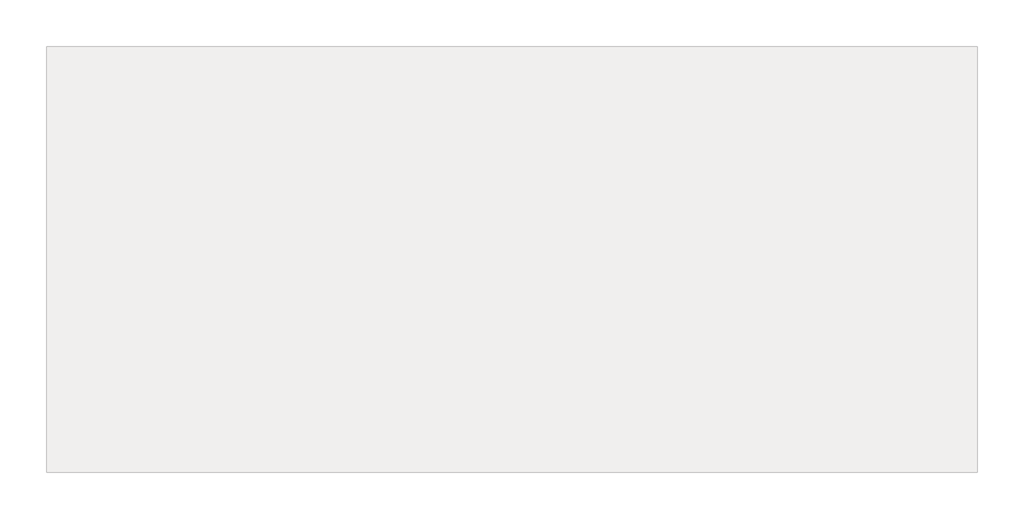
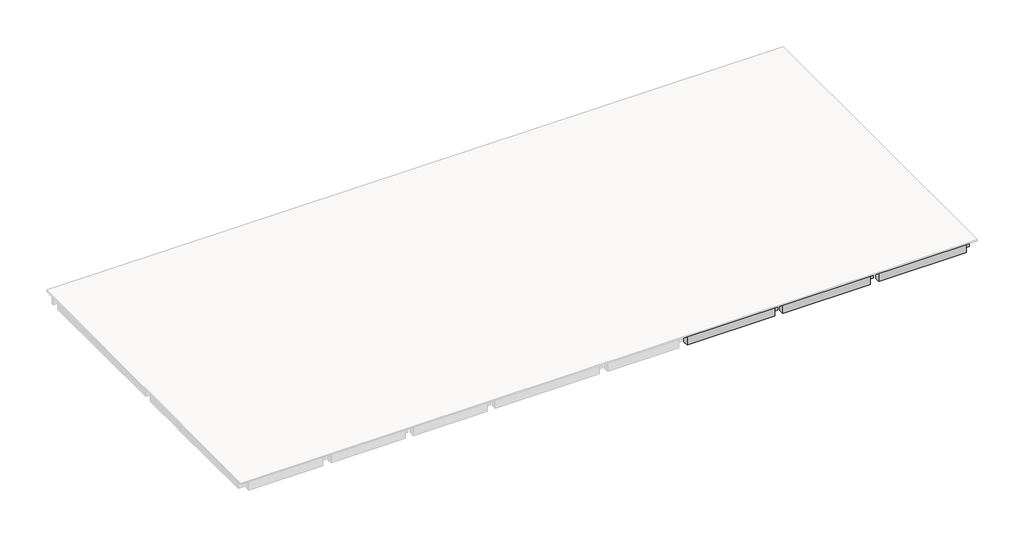
# One storey, part 2 of 2: 30 beams.
"""IFC4 building model written with IfcOpenShell, lengths in millimetres."""

from ifc_helpers import new_model, si_unit, frame, origin, place, context, project, spatial, polyline, outline, extrude, faceted_brep, element, save

model = new_model("IFC4")

# Units and contexts
model_context = context("Model", 3, world=origin())
ifc_project = project(units=[si_unit("LENGTHUNIT", "METRE", prefix="MILLI")], contexts=[model_context])

# Site, building, storey
site = spatial("IfcSite", under=ifc_project)
building = spatial("IfcBuilding", under=site)
storey = spatial("IfcBuildingStorey", under=building, Name="TOC", Elevation=7650.0)

# Beams
placement = place(None, origin())
element("IfcBeam", 1, ObjectType="RC Beam_Rectangular : H_SB_ACB_B400xH900", at=placement, inside=storey, context=model_context, shape_type="Brep", body=[
    faceted_brep([(39124.7, 12116.5208589, 6750.0), (39124.7, 12116.5208589, 7549.0), (38724.7, 12116.5208589, 7549.0), (32124.7, 12116.5208589, 7549.0), (32124.7, 12116.5208589, 6750.0), (38724.7, 12116.5208589, 6750.0), (39124.7, 12516.5208589, 6750.0), (32124.7, 12516.5208589, 6750.0), (38724.7, 12516.5208589, 6750.0), (39124.7, 12516.5208589, 7549.0), (32124.7, 12516.5208589, 7549.0), (38724.7, 12516.5208589, 7549.0)], [[[0, 1, 2, 3, 4, 5]], [[6, 0, 5, 4, 7, 8]], [[9, 6, 8, 7, 10, 11]], [[1, 9, 11, 10, 3, 2]], [[0, 6, 9, 1]], [[4, 3, 10, 7]]]),
])
element("IfcBeam", 2, ObjectType="RC Beam_Rectangular : H_SB_ACB_B400xH900", at=placement, inside=storey, context=model_context, shape_type="Brep", body=[
    faceted_brep([(46124.7, 12116.5208589, 6750.0), (46124.7, 12116.5208589, 7549.0), (45724.7, 12116.5208589, 7549.0), (39124.7, 12116.5208589, 7549.0), (39124.7, 12116.5208589, 6750.0), (45724.7, 12116.5208589, 6750.0), (46124.7, 12516.5208589, 6750.0), (39124.7, 12516.5208589, 6750.0), (45724.7, 12516.5208589, 6750.0), (46124.7, 12516.5208589, 7549.0), (39124.7, 12516.5208589, 7549.0), (45724.7, 12516.5208589, 7549.0)], [[[0, 1, 2, 3, 4, 5]], [[6, 0, 5, 4, 7, 8]], [[9, 6, 8, 7, 10, 11]], [[1, 9, 11, 10, 3, 2]], [[0, 6, 9, 1]], [[4, 3, 10, 7]]]),
])
element("IfcBeam", 3, ObjectType="RC Beam_Rectangular : H_SB_ACB_B400xH900", at=placement, inside=storey, context=model_context, shape_type="Brep", body=[
    faceted_brep([(53124.7, 12116.5208589, 6750.0), (53124.7, 12116.5208589, 7549.0), (52724.7, 12116.5208589, 7549.0), (46124.7, 12116.5208589, 7549.0), (46124.7, 12116.5208589, 6750.0), (52724.7, 12116.5208589, 6750.0), (53124.7, 12516.5208589, 6750.0), (46124.7, 12516.5208589, 6750.0), (52724.7, 12516.5208589, 6750.0), (53124.7, 12516.5208589, 7549.0), (46124.7, 12516.5208589, 7549.0), (52724.7, 12516.5208589, 7549.0)], [[[0, 1, 2, 3, 4, 5]], [[6, 0, 5, 4, 7, 8]], [[9, 6, 8, 7, 10, 11]], [[1, 9, 11, 10, 3, 2]], [[0, 6, 9, 1]], [[4, 3, 10, 7]]]),
])
element("IfcBeam", 4, ObjectType="RC Beam_Rectangular : H_SB_ACB_B400xH900", at=placement, inside=storey, context=model_context, shape_type="SweptSolid", body=[
    extrude(outline(polyline([(7500.0, 224.7), (6750.0, 224.7), (6750.0, 5624.7), (7500.0, 5624.7), (7500.0, 5724.7), (7549.0, 5724.7), (7549.0, 124.7), (7500.0, 124.7), (7500.0, 224.7)])), frame((0.0, 23816.5208589, 0.0), z_axis=(0.0, 1.0, 0.0), x_axis=(0.0, 0.0, 1.0)), (0.0, 0.0, 1.0), 400.0),
])
element("IfcBeam", 5, ObjectType="RC Beam_Rectangular : H_SB_ACB_B400xH900", at=placement, inside=storey, context=model_context, shape_type="SweptSolid", body=[
    extrude(outline(polyline([(7500.0, 6224.7), (6750.0, 6224.7), (6750.0, 11624.7), (7500.0, 11624.7), (7500.0, 11724.7), (7549.0, 11724.7), (7549.0, 6124.7), (7500.0, 6124.7), (7500.0, 6224.7)])), frame((0.0, 23816.5208589, 0.0), z_axis=(0.0, 1.0, 0.0), x_axis=(0.0, 0.0, 1.0)), (0.0, 0.0, 1.0), 400.0),
])
element("IfcBeam", 6, ObjectType="RC Beam_Rectangular : H_SB_ACB_B400xH900", at=placement, inside=storey, context=model_context, shape_type="SweptSolid", body=[
    extrude(outline(polyline([(7500.0, 12224.7), (6750.0, 12224.7), (6750.0, 17624.7), (7500.0, 17624.7), (7500.0, 17724.7), (7549.0, 17724.7), (7549.0, 12124.7), (7500.0, 12124.7), (7500.0, 12224.7)])), frame((0.0, 23816.5208589, 0.0), z_axis=(0.0, 1.0, 0.0), x_axis=(0.0, 0.0, 1.0)), (0.0, 0.0, 1.0), 400.0),
])
element("IfcBeam", 7, ObjectType="RC Beam_Rectangular : H_SB_ACB_B400xH900", at=placement, inside=storey, context=model_context, shape_type="SweptSolid", body=[
    extrude(outline(polyline([(7500.0, 18224.7), (6750.0, 18224.7), (6750.0, 25824.7), (7500.0, 25824.7), (7500.0, 25924.7), (7549.0, 25924.7), (7549.0, 18124.7), (7500.0, 18124.7), (7500.0, 18224.7)])), frame((0.0, 23816.5208589, 0.0), z_axis=(0.0, 1.0, 0.0), x_axis=(0.0, 0.0, 1.0)), (0.0, 0.0, 1.0), 400.0),
])
element("IfcBeam", 8, ObjectType="RC Beam_Rectangular : H_SB_ACB_B400xH900", at=placement, inside=storey, context=model_context, shape_type="SweptSolid", body=[
    extrude(outline(polyline([(7500.0, 26424.7), (6750.0, 26424.7), (6750.0, 31624.7), (7500.0, 31624.7), (7500.0, 31724.7), (7549.0, 31724.7), (7549.0, 26324.7), (7500.0, 26324.7), (7500.0, 26424.7)])), frame((0.0, 23816.5208589, 0.0), z_axis=(0.0, 1.0, 0.0), x_axis=(0.0, 0.0, 1.0)), (0.0, 0.0, 1.0), 400.0),
])
element("IfcBeam", 9, ObjectType="RC Beam_Rectangular : H_SB_ACB_B400xH900", at=placement, inside=storey, context=model_context, shape_type="SweptSolid", body=[
    extrude(outline(polyline([(7500.0, 32224.7), (6750.0, 32224.7), (6750.0, 38624.7), (7500.0, 38624.7), (7500.0, 38724.7), (7549.0, 38724.7), (7549.0, 32124.7), (7500.0, 32124.7), (7500.0, 32224.7)])), frame((0.0, 23816.5208589, 0.0), z_axis=(0.0, 1.0, 0.0), x_axis=(0.0, 0.0, 1.0)), (0.0, 0.0, 1.0), 400.0),
])
element("IfcBeam", 10, ObjectType="RC Beam_Rectangular : H_SB_ACB_B400xH900", at=placement, inside=storey, context=model_context, shape_type="SweptSolid", body=[
    extrude(outline(polyline([(7500.0, 39224.7), (6750.0, 39224.7), (6750.0, 45624.7), (7500.0, 45624.7), (7500.0, 45724.7), (7549.0, 45724.7), (7549.0, 39124.7), (7500.0, 39124.7), (7500.0, 39224.7)])), frame((0.0, 23816.5208589, 0.0), z_axis=(0.0, 1.0, 0.0), x_axis=(0.0, 0.0, 1.0)), (0.0, 0.0, 1.0), 400.0),
])
element("IfcBeam", 11, ObjectType="RC Beam_Rectangular : H_SB_ACB_B400xH900", at=placement, inside=storey, context=model_context, shape_type="SweptSolid", body=[
    extrude(outline(polyline([(7500.0, 46224.7), (6750.0, 46224.7), (6750.0, 52624.7), (7500.0, 52624.7), (7500.0, 52724.7), (7549.0, 52724.7), (7549.0, 46124.7), (7500.0, 46124.7), (7500.0, 46224.7)])), frame((0.0, 23816.5208589, 0.0), z_axis=(0.0, 1.0, 0.0), x_axis=(0.0, 0.0, 1.0)), (0.0, 0.0, 1.0), 400.0),
])
element("IfcBeam", 12, ObjectType="RC Beam_Rectangular : H_SB_ACB_B400xH900", at=placement, inside=storey, context=model_context, shape_type="Brep", body=[
    faceted_brep([(32224.7, 8216.5208589, 7500.0), (32224.7, 8216.5208589, 6750.0), (38624.7, 8216.5208589, 6750.0), (38624.7, 8216.5208589, 7500.0), (38724.7, 8216.5208589, 7500.0), (39124.7, 8216.5208589, 7500.0), (39124.7, 8216.5208589, 7549.0), (38724.7, 8216.5208589, 7549.0), (32124.7, 8216.5208589, 7549.0), (32124.7, 8216.5208589, 7500.0), (32224.7, 8616.5208589, 6750.0), (38624.7, 8616.5208589, 6750.0), (32224.7, 8616.5208589, 7500.0), (32124.7, 8616.5208589, 7500.0), (32124.7, 8616.5208589, 7549.0), (38724.7, 8616.5208589, 7549.0), (39124.7, 8616.5208589, 7549.0), (39124.7, 8616.5208589, 7500.0), (38724.7, 8616.5208589, 7500.0), (38624.7, 8616.5208589, 7500.0)], [[[0, 1, 2, 3, 4, 5, 6, 7, 8, 9]], [[1, 10, 11, 2]], [[10, 12, 13, 14, 15, 16, 17, 18, 19, 11]], [[1, 0, 12, 10]], [[0, 9, 13, 12]], [[19, 3, 2, 11]], [[3, 19, 18, 17, 5, 4]], [[8, 7, 6, 16, 15, 14]], [[16, 6, 5, 17]], [[8, 14, 13, 9]]]),
])
element("IfcBeam", 13, ObjectType="RC Beam_Rectangular : H_SB_ACB_B400xH900", at=placement, inside=storey, context=model_context, shape_type="Brep", body=[
    faceted_brep([(39224.7, 8216.5208589, 7500.0), (39224.7, 8216.5208589, 6750.0), (45624.7, 8216.5208589, 6750.0), (45624.7, 8216.5208589, 7500.0), (45724.7, 8216.5208589, 7500.0), (46124.7, 8216.5208589, 7500.0), (46124.7, 8216.5208589, 7549.0), (45724.7, 8216.5208589, 7549.0), (39124.7, 8216.5208589, 7549.0), (39124.7, 8216.5208589, 7500.0), (39224.7, 8616.5208589, 6750.0), (45624.7, 8616.5208589, 6750.0), (39224.7, 8616.5208589, 7500.0), (39124.7, 8616.5208589, 7500.0), (39124.7, 8616.5208589, 7549.0), (45724.7, 8616.5208589, 7549.0), (46124.7, 8616.5208589, 7549.0), (46124.7, 8616.5208589, 7500.0), (45724.7, 8616.5208589, 7500.0), (45624.7, 8616.5208589, 7500.0)], [[[0, 1, 2, 3, 4, 5, 6, 7, 8, 9]], [[1, 10, 11, 2]], [[10, 12, 13, 14, 15, 16, 17, 18, 19, 11]], [[1, 0, 12, 10]], [[0, 9, 13, 12]], [[19, 3, 2, 11]], [[3, 19, 18, 17, 5, 4]], [[8, 7, 6, 16, 15, 14]], [[16, 6, 5, 17]], [[8, 14, 13, 9]]]),
])
element("IfcBeam", 14, ObjectType="RC Beam_Rectangular : H_SB_ACB_B400xH900", at=placement, inside=storey, context=model_context, shape_type="Brep", body=[
    faceted_brep([(46224.7, 8216.5208589, 7500.0), (46224.7, 8216.5208589, 6750.0), (52624.7, 8216.5208589, 6750.0), (52624.7, 8216.5208589, 7500.0), (52724.7, 8216.5208589, 7500.0), (53124.7, 8216.5208589, 7500.0), (53124.7, 8216.5208589, 7549.0), (52724.7, 8216.5208589, 7549.0), (46124.7, 8216.5208589, 7549.0), (46124.7, 8216.5208589, 7500.0), (46224.7, 8616.5208589, 6750.0), (52624.7, 8616.5208589, 6750.0), (46224.7, 8616.5208589, 7500.0), (46124.7, 8616.5208589, 7500.0), (46124.7, 8616.5208589, 7549.0), (52724.7, 8616.5208589, 7549.0), (53124.7, 8616.5208589, 7549.0), (53124.7, 8616.5208589, 7500.0), (52724.7, 8616.5208589, 7500.0), (52624.7, 8616.5208589, 7500.0)], [[[0, 1, 2, 3, 4, 5, 6, 7, 8, 9]], [[1, 10, 11, 2]], [[10, 12, 13, 14, 15, 16, 17, 18, 19, 11]], [[1, 0, 12, 10]], [[0, 9, 13, 12]], [[19, 3, 2, 11]], [[3, 19, 18, 17, 5, 4]], [[8, 7, 6, 16, 15, 14]], [[16, 6, 5, 17]], [[8, 14, 13, 9]]]),
])
element("IfcBeam", 15, ObjectType="RC Beam_Rectangular : H_SB_ACB_B400xH900", at=placement, inside=storey, context=model_context, shape_type="Brep", body=[
    faceted_brep([(32224.7, 416.5208589, 7500.0), (32224.7, 416.5208589, 6750.0), (38624.7, 416.5208589, 6750.0), (38624.7, 416.5208589, 7500.0), (39124.7, 416.5208589, 7500.0), (39124.7, 416.5208589, 7549.0), (32124.7, 416.5208589, 7549.0), (32124.7, 416.5208589, 7500.0), (32224.7, 816.5208589, 6750.0), (38624.7, 816.5208589, 6750.0), (32224.7, 816.5208589, 7500.0), (32124.7, 816.5208589, 7500.0), (32124.7, 816.5208589, 7549.0), (38724.7, 816.5208589, 7549.0), (39124.7, 816.5208589, 7549.0), (39124.7, 816.5208589, 7500.0), (38724.7, 816.5208589, 7500.0), (38624.7, 816.5208589, 7500.0)], [[[0, 1, 2, 3, 4, 5, 6, 7]], [[1, 8, 9, 2]], [[8, 10, 11, 12, 13, 14, 15, 16, 17, 9]], [[8, 1, 0, 10]], [[11, 10, 0, 7]], [[17, 3, 2, 9]], [[3, 17, 16, 15, 4]], [[6, 5, 14, 13, 12]], [[14, 5, 4, 15]], [[6, 12, 11, 7]]]),
])
element("IfcBeam", 16, ObjectType="RC Beam_Rectangular : H_SB_ACB_B400xH900", at=placement, inside=storey, context=model_context, shape_type="Brep", body=[
    faceted_brep([(39224.7, 416.5208589, 7500.0), (39224.7, 416.5208589, 6750.0), (45624.7, 416.5208589, 6750.0), (45624.7, 416.5208589, 7500.0), (46124.7, 416.5208589, 7500.0), (46124.7, 416.5208589, 7549.0), (39124.7, 416.5208589, 7549.0), (39124.7, 416.5208589, 7500.0), (39224.7, 816.5208589, 6750.0), (45624.7, 816.5208589, 6750.0), (39224.7, 816.5208589, 7500.0), (39124.7, 816.5208589, 7500.0), (39124.7, 816.5208589, 7549.0), (45724.7, 816.5208589, 7549.0), (46124.7, 816.5208589, 7549.0), (46124.7, 816.5208589, 7500.0), (45724.7, 816.5208589, 7500.0), (45624.7, 816.5208589, 7500.0)], [[[0, 1, 2, 3, 4, 5, 6, 7]], [[1, 8, 9, 2]], [[8, 10, 11, 12, 13, 14, 15, 16, 17, 9]], [[8, 1, 0, 10]], [[11, 10, 0, 7]], [[17, 3, 2, 9]], [[3, 17, 16, 15, 4]], [[6, 5, 14, 13, 12]], [[14, 5, 4, 15]], [[6, 12, 11, 7]]]),
])
element("IfcBeam", 17, ObjectType="RC Beam_Rectangular : H_SB_ACB_B400xH900", at=placement, inside=storey, context=model_context, shape_type="Brep", body=[
    faceted_brep([(46224.7, 416.5208589, 7500.0), (46224.7, 416.5208589, 6750.0), (52624.7, 416.5208589, 6750.0), (52624.7, 416.5208589, 7500.0), (53124.7, 416.5208589, 7500.0), (53124.7, 416.5208589, 7549.0), (46124.7, 416.5208589, 7549.0), (46124.7, 416.5208589, 7500.0), (46224.7, 816.5208589, 6750.0), (52624.7, 816.5208589, 6750.0), (46224.7, 816.5208589, 7500.0), (46124.7, 816.5208589, 7500.0), (46124.7, 816.5208589, 7549.0), (52724.7, 816.5208589, 7549.0), (53124.7, 816.5208589, 7549.0), (53124.7, 816.5208589, 7500.0), (52724.7, 816.5208589, 7500.0), (52624.7, 816.5208589, 7500.0)], [[[0, 1, 2, 3, 4, 5, 6, 7]], [[1, 8, 9, 2]], [[8, 10, 11, 12, 13, 14, 15, 16, 17, 9]], [[8, 1, 0, 10]], [[11, 10, 0, 7]], [[17, 3, 2, 9]], [[3, 17, 16, 15, 4]], [[6, 5, 14, 13, 12]], [[14, 5, 4, 15]], [[6, 12, 11, 7]]]),
])
element("IfcBeam", 18, ObjectType="RC Beam_Rectangular : H_SB_ACB_B400xH900", at=placement, inside=storey, context=model_context, shape_type="Brep", body=[
    faceted_brep([(12124.7, 24429.2208589, 6750.0), (11724.7, 24429.2208589, 6750.0), (11724.7, 24429.2208589, 7549.0), (12124.7, 24429.2208589, 7549.0), (12124.7, 12616.5208589, 7500.0), (12124.7, 12616.5208589, 6750.0), (12124.7, 23716.5208589, 6750.0), (12124.7, 23716.5208589, 7500.0), (12124.7, 23816.5208589, 7500.0), (12124.7, 24216.5208589, 7500.0), (12124.7, 24316.5208589, 7500.0), (12124.7, 24316.5208589, 6750.0), (12124.7, 24216.5208589, 7549.0), (12124.7, 23816.5208589, 7549.0), (12124.7, 12516.5208589, 7549.0), (12124.7, 12516.5208589, 7500.0), (11724.7, 24316.5208589, 6750.0), (11724.7, 24316.5208589, 7500.0), (11724.7, 24216.5208589, 7500.0), (11724.7, 23816.5208589, 7500.0), (11724.7, 23716.5208589, 7500.0), (11724.7, 23716.5208589, 6750.0), (11724.7, 12616.5208589, 6750.0), (11724.7, 12616.5208589, 7500.0), (11724.7, 12516.5208589, 7500.0), (11724.7, 12516.5208589, 7549.0), (11724.7, 23816.5208589, 7549.0), (11724.7, 24216.5208589, 7549.0)], [[[0, 1, 2, 3]], [[4, 5, 6, 7, 8, 9, 10, 11, 0, 3, 12, 13, 14, 15]], [[1, 0, 11, 16]], [[2, 1, 16, 17, 18, 19, 20, 21, 22, 23, 24, 25, 26, 27]], [[24, 15, 14, 25]], [[5, 4, 23, 22]], [[4, 15, 24, 23]], [[20, 7, 6, 21]], [[7, 20, 19, 18, 17, 10, 9, 8]], [[3, 2, 27, 26, 25, 14, 13, 12]], [[10, 17, 16, 11]], [[5, 22, 21, 6]]]),
])
element("IfcBeam", 19, ObjectType="RC Beam_Rectangular : H_SB_ACB_B400xH900", at=placement, inside=storey, context=model_context, shape_type="Brep", body=[
    faceted_brep([(18124.7, 24429.2208589, 6750.0), (17724.7, 24429.2208589, 6750.0), (17724.7, 24429.2208589, 7549.0), (18124.7, 24429.2208589, 7549.0), (18124.7, 12616.5208589, 7500.0), (18124.7, 12616.5208589, 6750.0), (18124.7, 23716.5208589, 6750.0), (18124.7, 23716.5208589, 7500.0), (18124.7, 23816.5208589, 7500.0), (18124.7, 24216.5208589, 7500.0), (18124.7, 24316.5208589, 7500.0), (18124.7, 24316.5208589, 6750.0), (18124.7, 24216.5208589, 7549.0), (18124.7, 23816.5208589, 7549.0), (18124.7, 12516.5208589, 7549.0), (18124.7, 12516.5208589, 7500.0), (17724.7, 24316.5208589, 6750.0), (17724.7, 24316.5208589, 7500.0), (17724.7, 24216.5208589, 7500.0), (17724.7, 23816.5208589, 7500.0), (17724.7, 23716.5208589, 7500.0), (17724.7, 23716.5208589, 6750.0), (17724.7, 12616.5208589, 6750.0), (17724.7, 12616.5208589, 7500.0), (17724.7, 12516.5208589, 7500.0), (17724.7, 12516.5208589, 7549.0), (17724.7, 23816.5208589, 7549.0), (17724.7, 24216.5208589, 7549.0)], [[[0, 1, 2, 3]], [[4, 5, 6, 7, 8, 9, 10, 11, 0, 3, 12, 13, 14, 15]], [[1, 0, 11, 16]], [[2, 1, 16, 17, 18, 19, 20, 21, 22, 23, 24, 25, 26, 27]], [[24, 15, 14, 25]], [[5, 4, 23, 22]], [[4, 15, 24, 23]], [[20, 7, 6, 21]], [[7, 20, 19, 18, 17, 10, 9, 8]], [[3, 2, 27, 26, 25, 14, 13, 12]], [[10, 17, 16, 11]], [[5, 22, 21, 6]]]),
])
element("IfcBeam", 20, ObjectType="RC Beam_Rectangular : H_SB_ACB_B400xH900", at=placement, inside=storey, context=model_context, shape_type="Brep", body=[
    faceted_brep([(26324.7, 24429.2208589, 6750.0), (25924.7, 24429.2208589, 6750.0), (25924.7, 24429.2208589, 7549.0), (26324.7, 24429.2208589, 7549.0), (26324.7, 24216.5208589, 7549.0), (26324.7, 23816.5208589, 7549.0), (26324.7, 12516.5208589, 7549.0), (26324.7, 12516.5208589, 6750.0), (26324.7, 23716.5208589, 6750.0), (26324.7, 23716.5208589, 7500.0), (26324.7, 23816.5208589, 7500.0), (26324.7, 24216.5208589, 7500.0), (26324.7, 24316.5208589, 7500.0), (26324.7, 24316.5208589, 6750.0), (25924.7, 24316.5208589, 6750.0), (25924.7, 12516.5208589, 6750.0), (25924.7, 12516.5208589, 7549.0), (25924.7, 23816.5208589, 7549.0), (25924.7, 24216.5208589, 7549.0), (25924.7, 24316.5208589, 7500.0), (25924.7, 24216.5208589, 7500.0), (25924.7, 23816.5208589, 7500.0), (25924.7, 23716.5208589, 7500.0), (25924.7, 23716.5208589, 6750.0)], [[[0, 1, 2, 3]], [[0, 3, 4, 5, 6, 7, 8, 9, 10, 11, 12, 13]], [[1, 0, 13, 14]], [[15, 16, 17, 18, 2, 1, 14, 19, 20, 21, 22, 23]], [[15, 7, 6, 16]], [[22, 9, 8, 23]], [[9, 22, 21, 20, 19, 12, 11, 10]], [[3, 2, 18, 17, 16, 6, 5, 4]], [[12, 19, 14, 13]], [[7, 15, 23, 8]]]),
])
element("IfcBeam", 21, ObjectType="RC Beam_Rectangular : H_SB_ACB_B400xH900", at=placement, inside=storey, context=model_context, shape_type="Brep", body=[
    faceted_brep([(32124.7, 24429.2208589, 6750.0), (31724.7, 24429.2208589, 6750.0), (31724.7, 24429.2208589, 7549.0), (32124.7, 24429.2208589, 7549.0), (32124.7, 24216.5208589, 7549.0), (32124.7, 23816.5208589, 7549.0), (32124.7, 12516.5208589, 7549.0), (32124.7, 12516.5208589, 6750.0), (32124.7, 23716.5208589, 6750.0), (32124.7, 23716.5208589, 7500.0), (32124.7, 23816.5208589, 7500.0), (32124.7, 24216.5208589, 7500.0), (32124.7, 24316.5208589, 7500.0), (32124.7, 24316.5208589, 6750.0), (31724.7, 24316.5208589, 6750.0), (31724.7, 12516.5208589, 6750.0), (31724.7, 12516.5208589, 7549.0), (31724.7, 23816.5208589, 7549.0), (31724.7, 24216.5208589, 7549.0), (31724.7, 24316.5208589, 7500.0), (31724.7, 24216.5208589, 7500.0), (31724.7, 23816.5208589, 7500.0), (31724.7, 23716.5208589, 7500.0), (31724.7, 23716.5208589, 6750.0)], [[[0, 1, 2, 3]], [[0, 3, 4, 5, 6, 7, 8, 9, 10, 11, 12, 13]], [[1, 0, 13, 14]], [[15, 16, 17, 18, 2, 1, 14, 19, 20, 21, 22, 23]], [[15, 7, 6, 16]], [[22, 9, 8, 23]], [[9, 22, 21, 20, 19, 12, 11, 10]], [[3, 2, 18, 17, 16, 6, 5, 4]], [[12, 19, 14, 13]], [[7, 15, 23, 8]]]),
])
element("IfcBeam", 22, ObjectType="RC Beam_Rectangular : H_SB_ACB_B400xH900", at=placement, inside=storey, context=model_context, shape_type="SweptSolid", body=[
    extrude(outline(polyline([(8116.5208589, 7500.0), (8116.5208589, 6750.0), (916.5208589, 6750.0), (916.5208589, 7500.0), (816.5208589, 7500.0), (816.5208589, 7549.0), (8216.5208589, 7549.0), (8216.5208589, 7500.0), (8116.5208589, 7500.0)])), frame((38724.7, 0.0, 0.0), z_axis=(1.0, 0.0, 0.0), x_axis=(0.0, 1.0, 0.0)), (0.0, 0.0, 1.0), 400.0),
])
element("IfcBeam", 23, ObjectType="RC Beam_Rectangular : H_SB_ACB_B400xH900", at=placement, inside=storey, context=model_context, shape_type="SweptSolid", body=[
    extrude(outline(polyline([(12116.5208589, 7549.0), (12116.5208589, 6750.0), (8716.5208589, 6750.0), (8716.5208589, 7500.0), (8616.5208589, 7500.0), (8616.5208589, 7549.0), (12116.5208589, 7549.0)])), frame((38724.7, 0.0, 0.0), z_axis=(1.0, 0.0, 0.0), x_axis=(0.0, 1.0, 0.0)), (0.0, 0.0, 1.0), 400.0),
])
element("IfcBeam", 24, ObjectType="RC Beam_Rectangular : H_SB_ACB_B400xH900", at=placement, inside=storey, context=model_context, shape_type="Brep", body=[
    faceted_brep([(39124.7, 24429.2208589, 6750.0), (38724.7, 24429.2208589, 6750.0), (38724.7, 24429.2208589, 7549.0), (39124.7, 24429.2208589, 7549.0), (39124.7, 24216.5208589, 7549.0), (39124.7, 23816.5208589, 7549.0), (39124.7, 12516.5208589, 7549.0), (39124.7, 12516.5208589, 6750.0), (39124.7, 23716.5208589, 6750.0), (39124.7, 23716.5208589, 7500.0), (39124.7, 23816.5208589, 7500.0), (39124.7, 24216.5208589, 7500.0), (39124.7, 24316.5208589, 7500.0), (39124.7, 24316.5208589, 6750.0), (38724.7, 24316.5208589, 6750.0), (38724.7, 12516.5208589, 6750.0), (38724.7, 12516.5208589, 7549.0), (38724.7, 23816.5208589, 7549.0), (38724.7, 24216.5208589, 7549.0), (38724.7, 24316.5208589, 7500.0), (38724.7, 24216.5208589, 7500.0), (38724.7, 23816.5208589, 7500.0), (38724.7, 23716.5208589, 7500.0), (38724.7, 23716.5208589, 6750.0)], [[[0, 1, 2, 3]], [[0, 3, 4, 5, 6, 7, 8, 9, 10, 11, 12, 13]], [[1, 0, 13, 14]], [[15, 16, 17, 18, 2, 1, 14, 19, 20, 21, 22, 23]], [[15, 7, 6, 16]], [[22, 9, 8, 23]], [[9, 22, 21, 20, 19, 12, 11, 10]], [[3, 2, 18, 17, 16, 6, 5, 4]], [[12, 19, 14, 13]], [[7, 15, 23, 8]]]),
])
element("IfcBeam", 25, ObjectType="RC Beam_Rectangular : H_SB_ACB_B400xH900", at=placement, inside=storey, context=model_context, shape_type="SweptSolid", body=[
    extrude(outline(polyline([(8116.5208589, 7500.0), (8116.5208589, 6750.0), (916.5208589, 6750.0), (916.5208589, 7500.0), (816.5208589, 7500.0), (816.5208589, 7549.0), (8216.5208589, 7549.0), (8216.5208589, 7500.0), (8116.5208589, 7500.0)])), frame((45724.7, 0.0, 0.0), z_axis=(1.0, 0.0, 0.0), x_axis=(0.0, 1.0, 0.0)), (0.0, 0.0, 1.0), 400.0),
])
element("IfcBeam", 26, ObjectType="RC Beam_Rectangular : H_SB_ACB_B400xH900", at=placement, inside=storey, context=model_context, shape_type="SweptSolid", body=[
    extrude(outline(polyline([(12116.5208589, 7549.0), (12116.5208589, 6750.0), (8716.5208589, 6750.0), (8716.5208589, 7500.0), (8616.5208589, 7500.0), (8616.5208589, 7549.0), (12116.5208589, 7549.0)])), frame((45724.7, 0.0, 0.0), z_axis=(1.0, 0.0, 0.0), x_axis=(0.0, 1.0, 0.0)), (0.0, 0.0, 1.0), 400.0),
])
element("IfcBeam", 27, ObjectType="RC Beam_Rectangular : H_SB_ACB_B400xH900", at=placement, inside=storey, context=model_context, shape_type="Brep", body=[
    faceted_brep([(46124.7, 24429.2208589, 6750.0), (45724.7, 24429.2208589, 6750.0), (45724.7, 24429.2208589, 7549.0), (46124.7, 24429.2208589, 7549.0), (46124.7, 24216.5208589, 7549.0), (46124.7, 23816.5208589, 7549.0), (46124.7, 12516.5208589, 7549.0), (46124.7, 12516.5208589, 6750.0), (46124.7, 23716.5208589, 6750.0), (46124.7, 23716.5208589, 7500.0), (46124.7, 23816.5208589, 7500.0), (46124.7, 24216.5208589, 7500.0), (46124.7, 24316.5208589, 7500.0), (46124.7, 24316.5208589, 6750.0), (45724.7, 24316.5208589, 6750.0), (45724.7, 12516.5208589, 6750.0), (45724.7, 12516.5208589, 7549.0), (45724.7, 23816.5208589, 7549.0), (45724.7, 24216.5208589, 7549.0), (45724.7, 24316.5208589, 7500.0), (45724.7, 24216.5208589, 7500.0), (45724.7, 23816.5208589, 7500.0), (45724.7, 23716.5208589, 7500.0), (45724.7, 23716.5208589, 6750.0)], [[[0, 1, 2, 3]], [[0, 3, 4, 5, 6, 7, 8, 9, 10, 11, 12, 13]], [[1, 0, 13, 14]], [[15, 16, 17, 18, 2, 1, 14, 19, 20, 21, 22, 23]], [[15, 7, 6, 16]], [[22, 9, 8, 23]], [[9, 22, 21, 20, 19, 12, 11, 10]], [[3, 2, 18, 17, 16, 6, 5, 4]], [[12, 19, 14, 13]], [[7, 15, 23, 8]]]),
])
element("IfcBeam", 28, ObjectType="RC Beam_Rectangular : H_SB_ACB_B400xH900", at=placement, inside=storey, context=model_context, shape_type="SweptSolid", body=[
    extrude(outline(polyline([(8116.5208589, 7500.0), (8116.5208589, 6750.0), (916.5208589, 6750.0), (916.5208589, 7500.0), (816.5208589, 7500.0), (816.5208589, 7549.0), (8216.5208589, 7549.0), (8216.5208589, 7500.0), (8116.5208589, 7500.0)])), frame((52724.7, 0.0, 0.0), z_axis=(1.0, 0.0, 0.0), x_axis=(0.0, 1.0, 0.0)), (0.0, 0.0, 1.0), 400.0),
])
element("IfcBeam", 29, ObjectType="RC Beam_Rectangular : H_SB_ACB_B400xH900", at=placement, inside=storey, context=model_context, shape_type="SweptSolid", body=[
    extrude(outline(polyline([(12116.5208589, 7549.0), (12116.5208589, 6750.0), (8716.5208589, 6750.0), (8716.5208589, 7500.0), (8616.5208589, 7500.0), (8616.5208589, 7549.0), (12116.5208589, 7549.0)])), frame((52724.7, 0.0, 0.0), z_axis=(1.0, 0.0, 0.0), x_axis=(0.0, 1.0, 0.0)), (0.0, 0.0, 1.0), 400.0),
])
element("IfcBeam", 30, ObjectType="RC Beam_Rectangular : H_SB_ACB_B400xH900", at=placement, inside=storey, context=model_context, shape_type="Brep", body=[
    faceted_brep([(53124.7, 24429.2208589, 6750.0), (52724.7, 24429.2208589, 6750.0), (52724.7, 24429.2208589, 7549.0), (53124.7, 24429.2208589, 7549.0), (53124.7, 23716.5208589, 6750.0), (53124.7, 23716.5208589, 7500.0), (53124.7, 24316.5208589, 7500.0), (53124.7, 24316.5208589, 6750.0), (53124.7, 12516.5208589, 7549.0), (53124.7, 12516.5208589, 6750.0), (52724.7, 24316.5208589, 6750.0), (52724.7, 24316.5208589, 7500.0), (52724.7, 24216.5208589, 7500.0), (52724.7, 23816.5208589, 7500.0), (52724.7, 23716.5208589, 7500.0), (52724.7, 23716.5208589, 6750.0), (52724.7, 12516.5208589, 6750.0), (52724.7, 12516.5208589, 7549.0), (52724.7, 23816.5208589, 7549.0), (52724.7, 24216.5208589, 7549.0)], [[[0, 1, 2, 3]], [[4, 5, 6, 7, 0, 3, 8, 9]], [[1, 0, 7, 10]], [[11, 12, 13, 14, 15, 16, 17, 18, 19, 2, 1, 10]], [[4, 15, 14, 5]], [[14, 13, 12, 11, 6, 5]], [[9, 8, 17, 16]], [[3, 2, 19, 18, 17, 8]], [[6, 11, 10, 7]], [[15, 4, 9, 16]]]),
])

save(model, "model.ifc")

# Revit data of these elements
# Type "RC Beam_Rectangular : H_SB_ACB_B400xH900"
#   중앙부 하부근 = ""
#   중앙부 상부근 = ""
#   중앙부 보조근 = ""
#   중앙부 늑근 = ""
#   외단부 하부근 = ""
#   외단부 상부근 = ""
#   외단부 보조근 = ""
#   외단부 늑근 = ""
#   부호 = "TG3"
#   내단부 하부근 = ""
#   내단부 상부근 = ""
#   내단부 보조근 = ""
#   내단부 늑근 = ""
#   ALL 하부근 = "3-D20"
#   ALL 상부근 = "3-D20"
#   ALL 보조근 = ""
#   ALL 늑근 = "2-D10 @120"
#   Width = 400.000 mm
#   Height = 900.000 mm
#   Length [instance default] = 1524.000 mm
#   b = 400.000 mm
#   h = 900.000 mm
#   hec_material3 [instance default] = none
#   hec_material2 [instance default] = none
#   hec_material1 [instance default] = none
#   Structural Material [instance default] = none
#   Assembly Code = ""
# Elements 1, 2, 3, 4, 5, 6, 7, 8, 9, 10, 11, 12, 13, 14, 15, 16, 17, 18, 19, 20, 21, 22, 23, 24, 25, 26, 27, 28, 29, 30 (IfcBeam, "RC Beam_Rectangular : H_SB_ACB_B400xH900")
#   hec_material3 = none
#   hec_material2 = none
#   hec_material1 = none
#   Structural Material = none
#   Phase Created = New Construction
